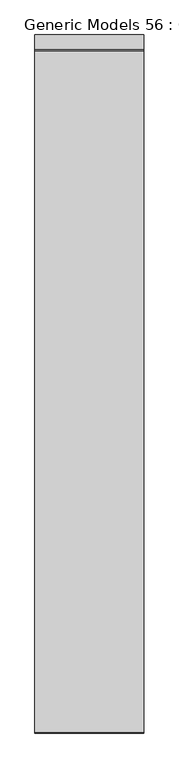
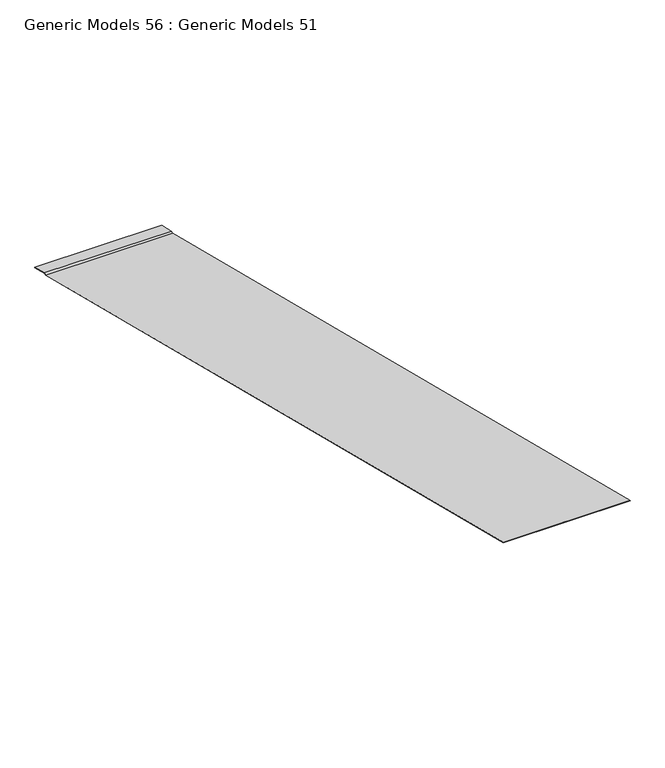
"""IFC4 building model written with IfcOpenShell, lengths in millimetres: proxy geometry, Generic Models 56 : Generic Models 51."""

from ifc_helpers import new_model, si_unit, frame, origin, place, context, project, spatial, polyline, outline, extrude, source, transform, mapped, element, save


def generic_models_56_generic_models_51_7569cca8(model_context):
    return source(origin(), model_context, "Body", "SweptSolid", [
        extrude(outline(polyline([(12300.7728751, 129660.1003293), (12307.1190749, 129661.8007884), (12346.7745512, 129651.8869194), (12346.5820385, 129651.1168687), (12307.1259708, 129660.9808857), (12300.7797709, 129659.2804266), (10394.8360209, 130135.7663641), (10395.0285336, 130136.5364147), (12300.7728751, 129660.1003293)])), frame((1084.7910488, 0.0, 0.0), z_axis=(1.0, 0.0, 0.0), x_axis=(0.0, 1.0, 0.0)), (0.0, 0.0, 1.0), 304.8),
    ])


if __name__ == "__main__":
    model = new_model("IFC4")
    model_context = context("Model", 3, world=origin())
    ifc_project = project(units=[si_unit("LENGTHUNIT", "METRE", prefix="MILLI")], contexts=[model_context])
    site = spatial("IfcSite", under=ifc_project)
    building = spatial("IfcBuilding", under=site)
    placement = place(None, origin())
    generic_models_56_generic_models_51_shape = generic_models_56_generic_models_51_7569cca8(model_context)
    element("IfcBuildingElementProxy", 1, Name="Generic Models 56 : Generic Models 51", ObjectType="Generic Models 56 : Generic Models 51", at=placement, inside=building, context=model_context, shape_type="MappedRepresentation", body=[
        mapped(generic_models_56_generic_models_51_shape, transform((0.0, 0.0, 0.0), x_axis=(1.0, 0.0, 0.0), y_axis=(0.0, 1.0, 0.0), z_axis=(0.0, 0.0, 1.0))),
    ])
    save(model, "model.ifc")

# Revit data of these elements
# Element 1 (IfcBuildingElementProxy, "Generic Models 56 : Generic Models 51")
#   Materials on its faces: "_(2) LAYERS NO. 30 ASTM D226 ASPHALT SATURATED ORGANIC FELT @ ROOF"
# Materials
#   "_(2) LAYERS NO. 30 ASTM D226 ASPHALT SATURATED ORGANIC FELT @ ROOF": class "Generic", colour RGB 67 154 161, transparency 0, Cost = 0
